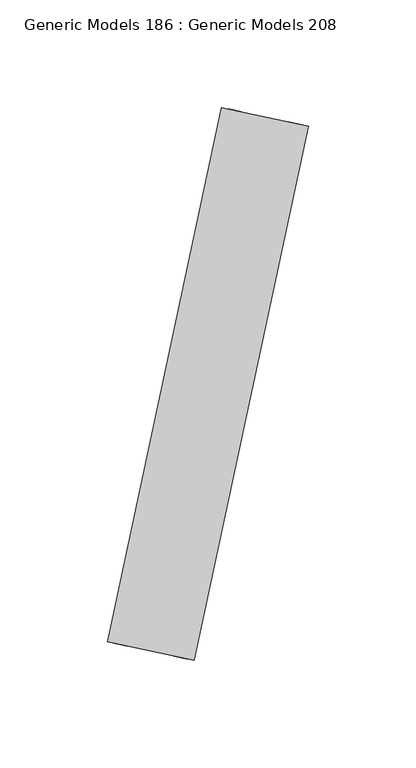
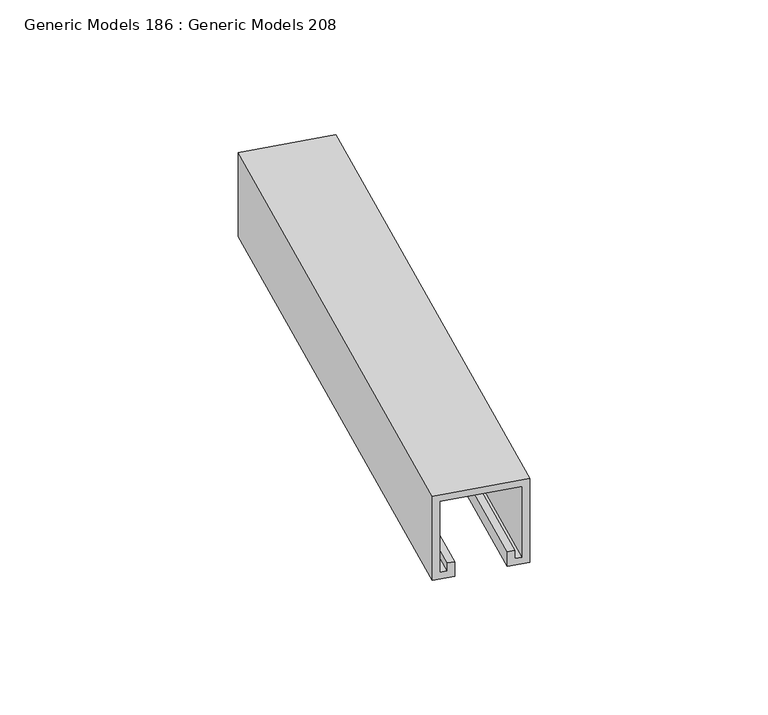
"""IFC4 building model written with IfcOpenShell, lengths in millimetres: proxy geometry, Generic Models 186 : Generic Models 208."""

from ifc_helpers import new_model, si_unit, frame, origin, place, context, project, spatial, polyline, outline, extrude, source, transform, mapped, element, save


def generic_models_186_generic_models_208_b3f29cbc(model_context):
    return source(origin(), model_context, "Body", "SweptSolid", [
        extrude(outline(polyline([(-3.175, 0.0), (-3.175, 34.925), (-38.1, 34.925), (-38.1, 31.75), (-34.13125, 31.75), (-34.13125, 28.575), (-41.275, 28.575), (-41.275, 38.1), (0.0, 38.1), (0.0, -3.1750001), (-41.275, -3.1750001), (-41.275, 6.35), (-34.13125, 6.35), (-34.13125, 3.175), (-38.1, 3.175), (-38.1, 0.0), (-3.175, 0.0)])), frame((-255.0543223, -22357.9169069, 1035.05), z_axis=(0.20919699342267242, 0.9778735183769496, 0.0), x_axis=(0.0, 0.0, 1.0)), (0.0, 0.0, 1.0), 254.0),
    ])


if __name__ == "__main__":
    model = new_model("IFC4")
    model_context = context("Model", 3, world=origin())
    ifc_project = project(units=[si_unit("LENGTHUNIT", "METRE", prefix="MILLI")], contexts=[model_context])
    site = spatial("IfcSite", under=ifc_project)
    building = spatial("IfcBuilding", under=site)
    placement = place(None, origin())
    generic_models_186_generic_models_208_shape = generic_models_186_generic_models_208_b3f29cbc(model_context)
    element("IfcBuildingElementProxy", 1, Name="Generic Models 186 : Generic Models 208", ObjectType="Generic Models 186 : Generic Models 208", at=placement, inside=building, context=model_context, shape_type="MappedRepresentation", body=[
        mapped(generic_models_186_generic_models_208_shape, transform((0.0, 0.0, 0.0), x_axis=(1.0, 0.0, 0.0), y_axis=(0.0, 1.0, 0.0), z_axis=(0.0, 0.0, 1.0))),
    ])
    save(model, "model.ifc")

# Revit data of these elements
# Element 1 (IfcBuildingElementProxy, "Generic Models 186 : Generic Models 208")
#   Materials on its faces: "UNISTRUT P1000, 1 5/8\" X 1 5/8\", CHANNEL OR ALUM. CHANNEL"
# Materials
#   "UNISTRUT P1000, 1 5/8\" X 1 5/8\", CHANNEL OR ALUM. CHANNEL": class "Metal", colour RGB 244 244 244, transparency 0, Description = "Aluminum 6061", Cost = 0
